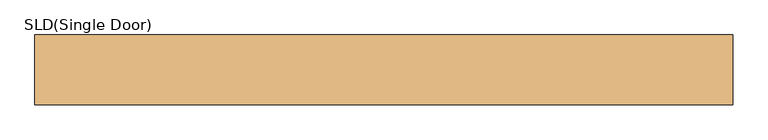
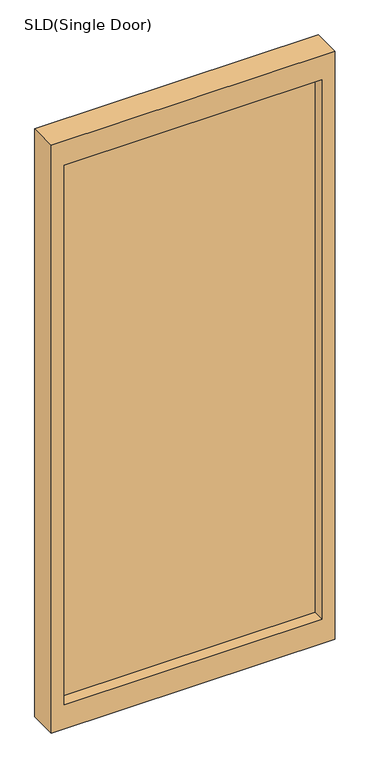
"""IFC4 building model written with IfcOpenShell, lengths in millimetres: door geometry, SLD(Single Door) : H_DR_AR B12_Door_Single_Glass_W980xH2200_SLD-1."""

from ifc_helpers import new_model, si_unit, frame, origin, place, context, project, spatial, polyline, outline, extrude, source, transform, mapped, element, save


def sld_single_door_cfd914d0(model_context):
    return source(origin(), model_context, "Body", "SweptSolid", [
        extrude(outline(polyline([(-55.0, -163.0), (-965.0, -163.0), (-965.0, -147.0), (-55.0, -147.0), (-55.0, -163.0)])), frame((0.0, 0.0, 90.0), z_axis=(0.0, 0.0, 1.0), x_axis=(1.0, 0.0, 0.0)), (0.0, 0.0, 1.0), 2010.0),
        extrude(outline(polyline([(2190.0, -10.0), (2190.0, -1010.0), (0.0, -1010.0), (0.0, -10.0), (2190.0, -10.0)]), holes=[polyline([(2100.0, -55.0), (90.0, -55.0), (90.0, -965.0), (2100.0, -965.0), (2100.0, -55.0)])]), frame((0.0, -205.0, 0.0), z_axis=(0.0, 1.0, 0.0), x_axis=(0.0, 0.0, 1.0)), (0.0, 0.0, 1.0), 100.0),
    ])


if __name__ == "__main__":
    model = new_model("IFC4")
    model_context = context("Model", 3, world=origin())
    ifc_project = project(units=[si_unit("LENGTHUNIT", "METRE", prefix="MILLI")], contexts=[model_context])
    site = spatial("IfcSite", under=ifc_project)
    building = spatial("IfcBuilding", under=site)
    placement = place(None, origin())
    sld_single_door_shape = sld_single_door_cfd914d0(model_context)
    element("IfcDoor", 1, ObjectType="SLD(Single Door) : H_DR_AR B12_Door_Single_Glass_W980xH2200_SLD-1", at=placement, inside=building, context=model_context, shape_type="MappedRepresentation", body=[
        mapped(sld_single_door_shape, transform((0.0, 0.0, 0.0), x_axis=(1.0, 0.0, 0.0), y_axis=(0.0, 1.0, 0.0), z_axis=(0.0, 0.0, 1.0))),
    ])
    save(model, "model.ifc")

# Revit data of these elements
# Type "SLD(Single Door) : H_DR_AR B12_Door_Single_Glass_W980xH2200_SLD-1"
#   Type Mark = "456"
#   Type Comments = "PD"
#   Analytic Construction = "<None>"
#   Thickness = 45 mm
#   Frame Projection Ext. = 25 mm
#   Frame Projection Int. = 25 mm
#   Frame Width = 75 mm
#   Height = 2200 mm
#   Width = 1020 mm
#   Door Width = 1000 mm
#   Door Frame Thk = 100 mm
#   Center [instance default] = 93 mm
#   Define Thermal Properties by = 1
#   Function = (empty or 0)
#   Wall Closure = (empty or 0)
# Element 1 (IfcDoor, "SLD(Single Door) : H_DR_AR B12_Door_Single_Glass_W980xH2200_SLD-1")
#   Center = 105 mm
#   Materials on its faces: "00_Metal_Stainless Steel", "00_Glass_Glass"
# Materials
#   "00_Metal_Stainless Steel": class "Metal", colour RGB 148 148 148, transparency 0, Description = "Steel", Cost = 0
#   "00_Glass_Glass": class "Glass", colour RGB 218 227 224, transparency 0.85, Description = "Glass", Cost = 0, Image = none
